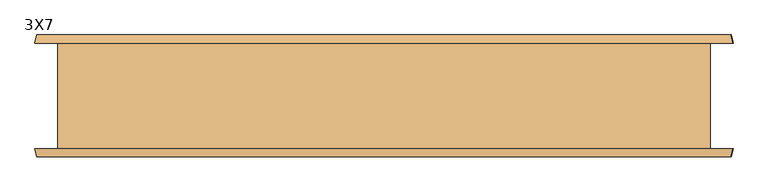
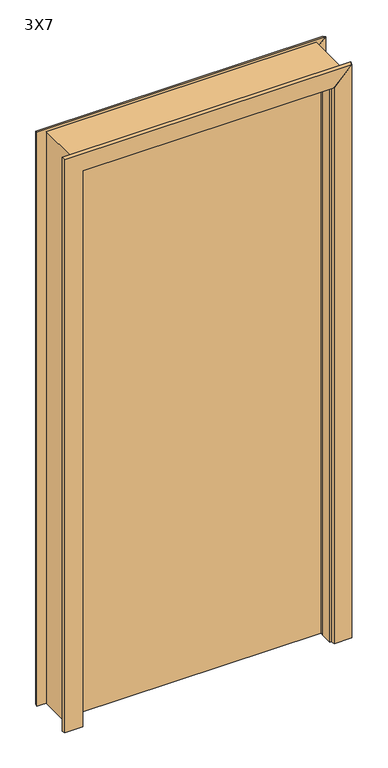
"""IFC4 building model written with IfcOpenShell, lengths in millimetres: door geometry, ASSA ABLOY BE_Doorset_Double Action Door_HardwareSet Info : 3X7."""

import ifcopenshell
import ifcopenshell.guid

model = None  # the IFC model being written
_history = None  # IfcOwnerHistory: only IFC2X3 demands one
_inside = {}  # id of a spatial element -> (the spatial element, [elements in it])
_under = {}  # id of a project, library or spatial element -> (it, [spatial elements below it])
_declared = {}  # id of a project -> (the project, [libraries it declares])
_typed = {}  # id of a type object -> (the type object, [elements of that type])
_made_of = {}  # id of a material, layer set ... -> (it, [elements and type objects made of it])


def new_model(schema):
    """Start an empty IFC model of exactly this schema.

    Asked for "IFC4X3", IfcOpenShell would pick the latest addendum, in which some entities
    have other attributes; the version numbers below select the first issue.
    IFC2X3 requires an IfcOwnerHistory on every rooted entity: one is made here for all.
    """
    global model, _history
    if schema == "IFC4X3":
        model = ifcopenshell.file(schema_version=(4, 3, 0, 0))
    else:
        model = ifcopenshell.file(schema=schema)
    _inside.clear()
    _under.clear()
    _declared.clear()
    _typed.clear()
    _made_of.clear()
    _history = None
    if model.schema == "IFC2X3":
        org = make("IfcOrganization", Name="unknown")
        user = make(
            "IfcPersonAndOrganization",
            ThePerson=make("IfcPerson", FamilyName="unknown"),
            TheOrganization=org,
        )
        app = make(
            "IfcApplication",
            ApplicationDeveloper=org,
            Version="unknown",
            ApplicationFullName="unknown",
            ApplicationIdentifier="unknown",
        )
        _history = make(
            "IfcOwnerHistory",
            OwningUser=user,
            OwningApplication=app,
            ChangeAction="ADDED",
            CreationDate=0,
        )
    return model


def make(cls, **values):
    """One entity of the class cls with the attributes given. An attribute that is None is left unset."""
    return model.create_entity(
        cls, **{name: value for name, value in values.items() if value is not None}
    )


def rooted(cls, **values):
    """An entity with a GlobalId (a new one), such as an element, a storey or a relation."""
    return make(cls, GlobalId=ifcopenshell.guid.new(), OwnerHistory=_history, **values)


def si_unit(unit_type, name, prefix=None):
    """IfcSIUnit, for example si_unit("LENGTHUNIT", "METRE", prefix="MILLI")."""
    return make("IfcSIUnit", UnitType=unit_type, Prefix=prefix, Name=name)


def assignment(units):
    """IfcUnitAssignment: the units of a project."""
    return None if units is None else make("IfcUnitAssignment", Units=units)


def point(xyz):
    """IfcCartesianPoint."""
    return None if xyz is None else make("IfcCartesianPoint", Coordinates=xyz)


def direction(xyz):
    """IfcDirection."""
    return None if xyz is None else make("IfcDirection", DirectionRatios=xyz)


def frame(location, z_axis=None, x_axis=None):
    """IfcAxis2Placement3D, a coordinate frame: its origin and axes. An axis left out is left unset."""
    return make(
        "IfcAxis2Placement3D",
        Location=point(location),
        Axis=direction(z_axis),
        RefDirection=direction(x_axis),
    )


def frame_2d(location, x_axis=None):
    """IfcAxis2Placement2D, a coordinate frame in the plane: its origin and x axis."""
    return make(
        "IfcAxis2Placement2D", Location=point(location), RefDirection=direction(x_axis)
    )


def origin():
    """The frame at (0, 0, 0) with its axes left unset."""
    return frame((0.0, 0.0, 0.0))


def place(relative_to, where):
    """IfcLocalPlacement: puts the frame where relative to a parent placement (None: the world)."""
    return make(
        "IfcLocalPlacement", PlacementRelTo=relative_to, RelativePlacement=where
    )


def context(
    kind, dimensions, precision=None, world=None, true_north=None, identifier=None
):
    """IfcGeometricRepresentationContext, for example the 3D "Model" context."""
    return make(
        "IfcGeometricRepresentationContext",
        ContextIdentifier=identifier,
        ContextType=kind,
        CoordinateSpaceDimension=dimensions,
        Precision=precision,
        WorldCoordinateSystem=world,
        TrueNorth=true_north,
    )


def project(units=None, contexts=None):
    """IfcProject with its units and contexts."""
    return rooted(
        "IfcProject",
        Name="project",
        RepresentationContexts=contexts,
        UnitsInContext=assignment(units),
    )


def spatial(cls, under=None, at=None, **own):
    """A site, building, storey or space (cls), placed at a placement, below another one or the project."""
    s = rooted(cls, ObjectPlacement=at, **own)
    if under is not None:
        _under.setdefault(under.id(), (under, []))[1].append(s)
    return s


def polyline(points):
    """IfcPolyline through the points."""
    return make("IfcPolyline", Points=[point(p) for p in points])


def circle_curve(where, radius):
    """IfcCircle in the frame where."""
    return make("IfcCircle", Position=where, Radius=radius)


def ellipse_curve(where, semi_axis1, semi_axis2):
    """IfcEllipse in the frame where."""
    return make(
        "IfcEllipse", Position=where, SemiAxis1=semi_axis1, SemiAxis2=semi_axis2
    )


def trimmed(basis, trim1, trim2, sense, master):
    """IfcTrimmedCurve: the piece of a basis curve between two trims."""
    return make(
        "IfcTrimmedCurve",
        BasisCurve=basis,
        Trim1=trim1,
        Trim2=trim2,
        SenseAgreement=sense,
        MasterRepresentation=master,
    )


def segment(curve, same_sense, transition):
    """IfcCompositeCurveSegment."""
    return make(
        "IfcCompositeCurveSegment",
        Transition=transition,
        SameSense=same_sense,
        ParentCurve=curve,
    )


def composite_curve(segments, self_intersect=None):
    """IfcCompositeCurve: segments joined end to end."""
    return make("IfcCompositeCurve", Segments=segments, SelfIntersect=self_intersect)


def outline(outer, holes=None, kind="AREA"):
    """IfcArbitraryClosedProfileDef: a profile drawn as a closed curve; with holes, ...WithVoids."""
    if holes is None:
        return make("IfcArbitraryClosedProfileDef", ProfileType=kind, OuterCurve=outer)
    return make(
        "IfcArbitraryProfileDefWithVoids",
        ProfileType=kind,
        OuterCurve=outer,
        InnerCurves=holes,
    )


def extrude(swept, where, along, depth):
    """IfcExtrudedAreaSolid: the profile swept, set in the frame where, extruded along a direction by depth."""
    return make(
        "IfcExtrudedAreaSolid",
        SweptArea=swept,
        Position=where,
        ExtrudedDirection=direction(along),
        Depth=depth,
    )


def faces_of(points, faces, orient=None, outer=None):
    """IfcFace entities. A face is a list of loops; a loop is a list of indices into points, from 0.

    orient and outer hold one flag for each loop. By default every Orientation is true, the
    first loop of a face is its IfcFaceOuterBound and the others are IfcFaceBound.
    """
    made = []
    for i, loops in enumerate(faces):
        bounds = []
        for j, loop in enumerate(loops):
            is_outer = j == 0 if outer is None else outer[i][j]
            bounds.append(
                make(
                    "IfcFaceOuterBound" if is_outer else "IfcFaceBound",
                    Bound=make("IfcPolyLoop", Polygon=[points[k] for k in loop]),
                    Orientation=True if orient is None else orient[i][j],
                )
            )
        made.append(make("IfcFace", Bounds=bounds))
    return made


def faceted_brep(points, faces, orient=None, outer=None, voids=None):
    """IfcFacetedBrep: a solid bounded by flat faces; with voids (closed shells), ...WithVoids."""
    shared = [point(p) for p in points]
    hull = make("IfcClosedShell", CfsFaces=faces_of(shared, faces, orient, outer))
    if voids is None:
        return make("IfcFacetedBrep", Outer=hull)
    return make(
        "IfcFacetedBrepWithVoids",
        Outer=hull,
        Voids=[
            make(cls, CfsFaces=faces_of(shared, fs, o, b)) for cls, fs, o, b in voids
        ],
    )


def shape(context_of_items, identifier, shape_type, items):
    """IfcShapeRepresentation: the items that make up one representation, for example the "Body"."""
    return make(
        "IfcShapeRepresentation",
        ContextOfItems=context_of_items,
        RepresentationIdentifier=identifier,
        RepresentationType=shape_type,
        Items=items,
    )


def source(mapping_origin, context_of_items, identifier, shape_type, items):
    """IfcRepresentationMap: a shape defined once, which mapped items show again and again."""
    return make(
        "IfcRepresentationMap",
        MappingOrigin=mapping_origin,
        MappedRepresentation=shape(context_of_items, identifier, shape_type, items),
    )


def transform(
    local_origin,
    x_axis=None,
    y_axis=None,
    z_axis=None,
    scale=None,
    scale2=None,
    scale3=None,
    uniform=True,
):
    """IfcCartesianTransformationOperator3D, or its non-uniform kind. x_axis, y_axis, z_axis: its Axis1, 2, 3."""
    if uniform:
        return make(
            "IfcCartesianTransformationOperator3D",
            Axis1=direction(x_axis),
            Axis2=direction(y_axis),
            LocalOrigin=point(local_origin),
            Scale=scale,
            Axis3=direction(z_axis),
        )
    return make(
        "IfcCartesianTransformationOperator3DnonUniform",
        Axis1=direction(x_axis),
        Axis2=direction(y_axis),
        LocalOrigin=point(local_origin),
        Scale=scale,
        Axis3=direction(z_axis),
        Scale2=scale2,
        Scale3=scale3,
    )


def mapped(mapping_source, mapping_target):
    """IfcMappedItem: shows the shape of a source again, moved by a transform."""
    return make(
        "IfcMappedItem", MappingSource=mapping_source, MappingTarget=mapping_target
    )


def made_of(thing, what):
    """Note that an element or type object is made of a material, layer set ...; save() writes the relation."""
    if what is not None:
        _made_of.setdefault(what.id(), (what, []))[1].append(thing)
    return thing


def element(
    cls,
    number,
    at=None,
    inside=None,
    cuts=None,
    type_object=None,
    material=None,
    context=None,
    identifier="Body",
    shape_type=None,
    held_by="IfcProductDefinitionShape",
    body=None,
    shapes=None,
    **own,
):
    """One element of the class cls, such as IfcWall. Its Tag is "e" and its number.

    at: its placement. inside: the storey or other place that contains it. cuts: it is an
    opening in that element (IfcRelVoidsElement). A single representation is given by context,
    identifier, shape_type and body (its items); several are given by shapes. held_by: the class
    of the entity that holds the representations. save() writes the other relations.
    """
    e = rooted(cls, Tag="e%d" % number, ObjectPlacement=at, **own)
    if body is not None:
        shapes = [shape(context, identifier, shape_type, body)]
    if shapes is not None:
        e.Representation = make(held_by, Representations=shapes)
    if inside is not None:
        _inside.setdefault(inside.id(), (inside, []))[1].append(e)
    if cuts is not None:
        rooted(
            "IfcRelVoidsElement", RelatingBuildingElement=cuts, RelatedOpeningElement=e
        )
    if type_object is not None:
        _typed.setdefault(type_object.id(), (type_object, []))[1].append(e)
    return made_of(e, material)


def aggregate(whole, parts):
    """IfcRelAggregates: a whole, such as a stair, and the parts it consists of."""
    return rooted("IfcRelAggregates", RelatingObject=whole, RelatedObjects=parts)


def save(model, path):
    """Write the relations noted so far, then the file.

    IfcRelAggregates (storeys below a building ...), IfcRelContainedInSpatialStructure (elements
    in a storey), IfcRelDefinesByType, IfcRelAssociatesMaterial and IfcRelDeclares: one each for
    every whole, place, type object, material and project.
    """
    for whole, parts in _under.values():
        aggregate(whole, parts)
    for where, things in _inside.values():
        rooted(
            "IfcRelContainedInSpatialStructure",
            RelatedElements=things,
            RelatingStructure=where,
        )
    for kind, things in _typed.values():
        rooted("IfcRelDefinesByType", RelatedObjects=things, RelatingType=kind)
    for what, things in _made_of.values():
        rooted("IfcRelAssociatesMaterial", RelatedObjects=things, RelatingMaterial=what)
    for by, libraries in _declared.values():
        rooted("IfcRelDeclares", RelatingContext=by, RelatedDefinitions=libraries)
    model.write(path)


def plane_surface(at):
    """IfcPlane: the flat surface through the origin of the frame at, square to its z axis."""
    return make("IfcPlane", Position=at)


def revolved_surface(curve, axis_point, axis_direction):
    """IfcSurfaceOfRevolution: the curve turned about the line through axis_point along axis_direction."""
    return make(
        "IfcSurfaceOfRevolution",
        SweptCurve=make("IfcArbitraryOpenProfileDef", ProfileType="CURVE", Curve=curve),
        AxisPosition=make("IfcAxis1Placement", Location=point(axis_point), Axis=direction(axis_direction)),
    )


def advanced_brep(points, edges, surfaces, faces):
    """IfcAdvancedBrep: a solid bounded by faces that lie on surfaces and meet in shared edges.

    An edge is (start, end): straight between two places in points (the first is 0);
    or (start, end, curve); or (start, end, curve, False) where it runs against its curve.
    A face is (place in surfaces, loops), or (place, loops, False) where it looks against
    its surface's normal. A loop lists edges by number (the first is 1), with a minus sign
    where the edge is run from its end to its start. The first loop is the outer one.
    """
    corners = [point(p) for p in points]
    vertices = [make("IfcVertexPoint", VertexGeometry=c) for c in corners]
    made = []
    for start, end, *more in edges:
        made.append(
            make(
                "IfcEdgeCurve",
                EdgeStart=vertices[start],
                EdgeEnd=vertices[end],
                EdgeGeometry=more[0] if more else make("IfcPolyline", Points=[corners[start], corners[end]]),
                SameSense=more[1] if len(more) > 1 else True,
            )
        )
    hull = []
    for where, loops, *sense in faces:
        bounds = []
        for j, loop in enumerate(loops):
            ring = [make("IfcOrientedEdge", EdgeElement=made[abs(k) - 1], Orientation=k > 0) for k in loop]
            bounds.append(
                make(
                    "IfcFaceOuterBound" if j == 0 else "IfcFaceBound",
                    Bound=make("IfcEdgeLoop", EdgeList=ring),
                    Orientation=True,
                )
            )
        hull.append(make("IfcAdvancedFace", Bounds=bounds, FaceSurface=surfaces[where], SameSense=sense[0] if sense else True))
    return make("IfcAdvancedBrep", Outer=make("IfcClosedShell", CfsFaces=hull))


def door_3x7_79b046d8(model_context):
    return source(origin(), model_context, "Body", "SolidModel", [
        extrude(outline(composite_curve([segment(polyline([(430.8440078, -25.0), (-429.2, -25.0), (-429.2, 25.0), (430.8440078, 25.0)]), True, "CONTINUOUS"), segment(trimmed(circle_curve(frame_2d((376.3004472, 0.0)), 60.0), [point((430.8440078, 25.0))], [point((430.8440078, -25.0))], False, "CARTESIAN"), True, "CONTINUOUS")], self_intersect=False)), frame((0.0, 0.0, 4.0), z_axis=(0.0, 0.0, 1.0), x_axis=(1.0, 0.0, 0.0)), (0.0, 0.0, 1.0), 2096.0),
        advanced_brep(
        [(432.1999993, -29.0558097, 0.0), (432.2, 29.0558084, 0.0), (432.2, 76.2, 0.0), (437.2, 76.2, 0.0), (440.2, 88.2, 0.0), (502.2, 88.2, 0.0), (505.2, 76.2, 0.0), (457.2, 76.2, 0.0), (457.2, -76.2, 0.0), (505.2, -76.2, 0.0), (502.2, -88.2, 0.0), (440.2, -88.2, 0.0), (437.2, -76.2, 0.0), (432.1999993, -76.2, 0.0), (432.1999993, -76.2, 2049.9999993), (432.1999993, -29.0558097, 2049.9999993), (437.2, -76.2, 2055.0), (440.2, -88.2, 2058.0), (502.2, -88.2, 2120.0), (505.2, -76.2, 2123.0), (457.2, -76.2, 2075.0), (457.2, 76.2, 2075.0), (505.2, 76.2, 2123.0), (502.2, 88.2, 2120.0), (440.2, 88.2, 2058.0), (437.2, 76.2, 2055.0), (432.2, 76.2, 2050.0), (432.2, 29.0558084, 2050.0)],
        [
            (0, 1, circle_curve(frame((376.3004472, 0.0, 0.0), z_axis=(0.0, 0.0, 1.0), x_axis=(-1.0, 0.0, 0.0)), 63.0)),
            (1, 2),
            (2, 3),
            (3, 4),
            (4, 5),
            (5, 6),
            (6, 7),
            (7, 8),
            (8, 9),
            (9, 10),
            (10, 11),
            (11, 12),
            (12, 13),
            (13, 0),
            (13, 14),
            (14, 15),
            (15, 0),
            (12, 16),
            (16, 14),
            (11, 17),
            (17, 16),
            (10, 18),
            (18, 17),
            (9, 19),
            (19, 18),
            (8, 20),
            (20, 19),
            (7, 21),
            (21, 20),
            (6, 22),
            (22, 21),
            (5, 23),
            (23, 22),
            (4, 24),
            (24, 23),
            (3, 25),
            (25, 24),
            (2, 26),
            (26, 25),
            (1, 27),
            (27, 26),
            (15, 27, ellipse_curve(frame((376.3004472, 0.0, 1994.1004472), z_axis=(-0.7071067811865507, 0.0, 0.7071067811865445), x_axis=(0.7071067811865445, 0.0, 0.7071067811865505)), 89.0954544, 63.0)),
        ],
        [
            plane_surface(frame((457.2, -76.2, 0.0), z_axis=(0.0, 0.0, -1.0), x_axis=(0.0, 1.0, 0.0))),
            plane_surface(frame((432.1999993, -29.0558097, 0.0), z_axis=(-1.0, 0.0, 0.0), x_axis=(0.0, 0.0, 1.0))),
            plane_surface(frame((432.1999993, -76.2, 0.0), z_axis=(0.0, -1.0, 0.0), x_axis=(0.0, 0.0, 1.0))),
            plane_surface(frame((437.2, -76.2, 0.0), z_axis=(-0.9701425001453396, -0.24253562503630208, 0.0), x_axis=(0.0, 0.0, 1.0))),
            plane_surface(frame((440.2, -88.2, 0.0), z_axis=(0.0, -1.0, 0.0), x_axis=(0.0, 0.0, 1.0))),
            plane_surface(frame((502.2, -88.2, 0.0), z_axis=(0.9701425001453319, -0.24253562503633297, 0.0), x_axis=(0.0, 0.0, 1.0))),
            plane_surface(frame((505.2, -76.2, 0.0), z_axis=(0.0, 1.0, 0.0), x_axis=(0.0, 0.0, 1.0))),
            plane_surface(frame((457.2, -76.2, 0.0), z_axis=(1.0, 0.0, 0.0), x_axis=(0.0, 0.0, 1.0))),
            plane_surface(frame((457.2, 76.2, 0.0), z_axis=(0.0, -1.0, 0.0), x_axis=(0.0, 0.0, 1.0))),
            plane_surface(frame((505.2, 76.2, 0.0), z_axis=(0.9701425001453553, 0.24253562503623965, 0.0), x_axis=(0.0, 0.0, 1.0))),
            plane_surface(frame((502.2, 88.2, 0.0), z_axis=(0.0, 1.0, 0.0), x_axis=(0.0, 0.0, 1.0))),
            plane_surface(frame((440.2, 88.2, 0.0), z_axis=(-0.970142500145363, 0.24253562503620874, 0.0), x_axis=(0.0, 0.0, 1.0))),
            plane_surface(frame((437.2, 76.2, 0.0), z_axis=(0.0, 1.0, 0.0), x_axis=(0.0, 0.0, 1.0))),
            plane_surface(frame((432.2, 76.2, 0.0), z_axis=(-1.0, 0.0, 0.0), x_axis=(0.0, 0.0, 1.0))),
            revolved_surface(polyline([(313.3004472, 0.0, 2057.100447179137), (313.3004472, 0.0, 0.0)]), (376.3004472, 0.0, 0.0), (0.0, 0.0, 1.0)),
            plane_surface(frame((345.6190436, 88.2, 1963.4190436), z_axis=(-0.7071067811865507, 0.0, 0.7071067811865445), x_axis=(0.0, -1.0, 0.0))),
        ],
        [
            (0, [[1, 2, 3, 4, 5, 6, 7, 8, 9, 10, 11, 12, 13, 14]]),
            (1, [[15, 16, 17, -14]]),
            (2, [[18, 19, -15, -13]]),
            (3, [[20, 21, -18, -12]]),
            (4, [[22, 23, -20, -11]]),
            (5, [[24, 25, -22, -10]]),
            (6, [[26, 27, -24, -9]]),
            (7, [[28, 29, -26, -8]]),
            (8, [[30, 31, -28, -7]]),
            (9, [[32, 33, -30, -6]]),
            (10, [[34, 35, -32, -5]]),
            (11, [[36, 37, -34, -4]]),
            (12, [[38, 39, -36, -3]]),
            (13, [[40, 41, -38, -2]]),
            (14, [[-17, 42, -40, -1]]),
            (15, [[-19, -21, -23, -25, -27, -29, -31, -33, -35, -37, -39, -41, -42, -16]]),
        ],
    ),
        faceted_brep([(-432.1999993, 76.2, 0.0), (-432.1999993, -76.2, 0.0), (-437.2, -76.2, 0.0), (-440.2, -88.2, 0.0), (-502.2, -88.2, 0.0), (-505.2, -76.2, 0.0), (-457.2, -76.2, 0.0), (-457.2, 76.2, 0.0), (-505.2, 76.2, 0.0), (-502.2, 88.2, 0.0), (-440.2, 88.2, 0.0), (-437.2, 76.2, 0.0), (-437.2, 76.2, 2055.0), (437.2, 76.2, 2055.0), (432.1999993, 76.2, 2049.9999993), (-432.1999993, 76.2, 2049.9999993), (-440.2, 88.2, 2058.0), (-502.2, 88.2, 2120.0), (502.2, 88.2, 2120.0), (440.2, 88.2, 2058.0), (-505.2, 76.2, 2123.0), (-457.2, 76.2, 2075.0), (457.2, 76.2, 2075.0), (505.2, 76.2, 2123.0), (-457.2, -76.2, 2075.0), (-505.2, -76.2, 2123.0), (505.2, -76.2, 2123.0), (457.2, -76.2, 2075.0), (-502.2, -88.2, 2120.0), (-440.2, -88.2, 2058.0), (440.2, -88.2, 2058.0), (502.2, -88.2, 2120.0), (-437.2, -76.2, 2055.0), (-432.1999993, -76.2, 2049.9999993), (432.1999993, -76.2, 2049.9999993), (437.2, -76.2, 2055.0)], [[[0, 1, 2, 3, 4, 5, 6, 7, 8, 9, 10, 11]], [[11, 12, 13, 14, 15, 0]], [[10, 16, 12, 11]], [[9, 17, 18, 19, 16, 10]], [[8, 20, 17, 9]], [[7, 21, 22, 23, 20, 8]], [[6, 24, 21, 7]], [[5, 25, 26, 27, 24, 6]], [[4, 28, 25, 5]], [[3, 29, 30, 31, 28, 4]], [[2, 32, 29, 3]], [[1, 33, 34, 35, 32, 2]], [[0, 15, 33, 1]], [[15, 14, 34, 33]], [[32, 35, 30, 29]], [[28, 31, 26, 25]], [[24, 27, 22, 21]], [[23, 18, 17, 20]], [[16, 19, 13, 12]], [[14, 13, 19, 18, 23, 22, 27, 26, 31, 30, 35, 34]]]),
        extrude(outline(polyline([(0.0, -457.2), (2100.0, -457.2), (2100.0, 457.2), (0.0, 457.2), (0.0, 472.2), (2115.0, 472.2), (2115.0, -472.2), (0.0, -472.2), (0.0, -457.2)])), frame((0.0, -76.2, 0.0), z_axis=(0.0, 1.0, 0.0), x_axis=(0.0, 0.0, 1.0)), (0.0, 0.0, 1.0), 152.4),
    ])


if __name__ == "__main__":
    model = new_model("IFC4")
    model_context = context("Model", 3, world=origin())
    ifc_project = project(units=[si_unit("LENGTHUNIT", "METRE", prefix="MILLI")], contexts=[model_context])
    site = spatial("IfcSite", under=ifc_project)
    building = spatial("IfcBuilding", under=site)
    placement = place(None, origin())
    door_3x7_shape = door_3x7_79b046d8(model_context)
    element("IfcDoor", 1, ObjectType="ASSA ABLOY BE_Doorset_Double Action Door_HardwareSet Info : 3X7", at=placement, inside=building, context=model_context, shape_type="MappedRepresentation", body=[
        mapped(door_3x7_shape, transform((0.0, 0.0, 0.0), x_axis=(1.0, 0.0, 0.0), y_axis=(0.0, 1.0, 0.0), z_axis=(0.0, 0.0, 1.0))),
    ])
    save(model, "model.ifc")

# Revit data of these elements
# Type "ASSA ABLOY BE_Doorset_Double Action Door_HardwareSet Info : 3X7"
#   Type Mark = "45"
#   Uniclass 2.0 Description = "Doorsets"
#   Uniclass 2.0 Code = "PR-59-23"
#   Uniclass 1.4 Description = "Doors"
#   Uniclass 1.4 Code = "JL20"
#   URL = "http://www.assaabloy.be/door-solutions/double-action-door-solution"
#   UNSPSC Code = "301715"
#   Type Comments = "1380x2110 (1430X2135)"
#   Region Europe = "BE, LU"
#   Provider = "ASSA ABLOY Belgium"
#   Product Guid = "1d6185b8-f4a7-4cd1-8e4c-530cf6da835d"
#   OmniClass Description = "Doors"
#   OmniClass Code = "23-17 11 00"
#   Name = "Double Action Door Solution"
#   NBS Reference Description = "Doorsets"
#   NBS Reference Code = "59-23"
#   Model = "ASSA ABLOY BE_Doorset_Double Action Door_HardwareSet Info"
#   Manufacturer = "ASSA ABLOY"
#   Lock Cases = "A56D5_D5_by Litto ASSA ABLOY"
#   IFC Classification = "Door"
#   Hardware Set = "A-S-1-DC475-BE04"
#   Door Closers = "DC475_Cam-Motion®_by ASSA ABLOY"
#   Description = "The ASSA ABLOY Belgium solution for Interior double action self-closing door equipped with a Cam-Motion® Floor Spring for an easier opening. This solution can also be used for two-way movement fire rated doors."
#   Date of publishing = "2016-03-04"
#   Contact Provider = "http://www.assaabloy.be/contact-solutions-team"
#   BIMobject category = "Door Sets"
#   BIMobject Unique ref = "A-S-1-DC475-BE04"
#   BIMobject Product Page = "http://bimobject.com/en/assaabloy-be/product/A-S-1-DC475-BE04"
#   BIMobject Product Group = "Single-Wood-Self Closing"
#   BIMobject Product Family = "Interior Door Solutions"
#   BIMobject Instructions Video = "https://www.youtube.com/watch?v=sh1CO-2jNM0"
#   BIMobject Brand = "ASSA ABLOY BE"
#   Architectural and Accessory Hardware = "TL0452SS_TONIC LINE_by Litto ASSA ABLOY"
#   Analytic Construction = "<None>"
#   Min Door Width = 2' - 0.80315"
#   Min Door Height = 6' - 11.07087"
#   Max Door Width = 4' - 6.33071"
#   Max Door Height = 6' - 10.67717"
#   Thickness = 0' - 1.9685"
#   Rough Width = 3' - 1.1811"
#   Rough Height = 6' - 11.26772"
#   Height = 6' - 10.67717"
#   Width = 3' - 0"
#   Frame Depth [instance default] = 0' - 9.84252"
#   Door Panel Width = 2' - 10.4252"
#   Frame Width = 3' - 0"
#   Frame Height = 7' - 0"
#   Edition number = 1
#   Frame Material = Wood
#   Frame Finish = Light Grey
#   Door Material = Wood
#   Door Finish = Light Grey
#   Function = (empty or 0)
#   Wall Closure = (empty or 0)
# Element 1 (IfcDoor, "ASSA ABLOY BE_Doorset_Double Action Door_HardwareSet Info : 3X7")
#   Frame Depth = 0' - 6"
#   Materials on its faces: "Light Grey"
# Materials
#   "Wood": class "Generic", colour RGB 170 151 133, transparency 0, Cost = 0
#   "Light Grey": class "Unassigned", colour RGB 200 200 200, transparency 0, Cost = 0
